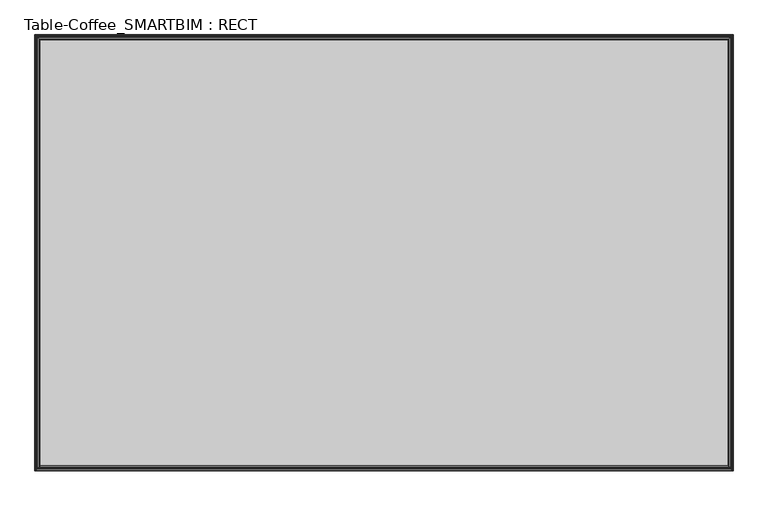
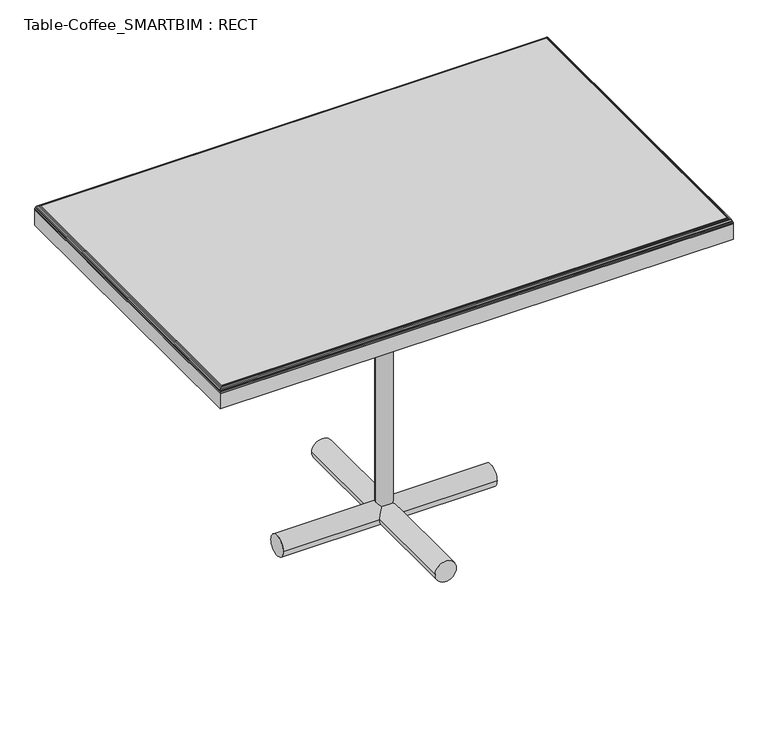
"""IFC4 building model written with IfcOpenShell, lengths in millimetres: furniture geometry, Table-Coffee_SMARTBIM : RECT."""

import ifcopenshell
import ifcopenshell.guid

model = None  # the IFC model being written
_history = None  # IfcOwnerHistory: only IFC2X3 demands one
_inside = {}  # id of a spatial element -> (the spatial element, [elements in it])
_under = {}  # id of a project, library or spatial element -> (it, [spatial elements below it])
_declared = {}  # id of a project -> (the project, [libraries it declares])
_typed = {}  # id of a type object -> (the type object, [elements of that type])
_made_of = {}  # id of a material, layer set ... -> (it, [elements and type objects made of it])


def new_model(schema):
    """Start an empty IFC model of exactly this schema.

    Asked for "IFC4X3", IfcOpenShell would pick the latest addendum, in which some entities
    have other attributes; the version numbers below select the first issue.
    IFC2X3 requires an IfcOwnerHistory on every rooted entity: one is made here for all.
    """
    global model, _history
    if schema == "IFC4X3":
        model = ifcopenshell.file(schema_version=(4, 3, 0, 0))
    else:
        model = ifcopenshell.file(schema=schema)
    _inside.clear()
    _under.clear()
    _declared.clear()
    _typed.clear()
    _made_of.clear()
    _history = None
    if model.schema == "IFC2X3":
        org = make("IfcOrganization", Name="unknown")
        user = make(
            "IfcPersonAndOrganization",
            ThePerson=make("IfcPerson", FamilyName="unknown"),
            TheOrganization=org,
        )
        app = make(
            "IfcApplication",
            ApplicationDeveloper=org,
            Version="unknown",
            ApplicationFullName="unknown",
            ApplicationIdentifier="unknown",
        )
        _history = make(
            "IfcOwnerHistory",
            OwningUser=user,
            OwningApplication=app,
            ChangeAction="ADDED",
            CreationDate=0,
        )
    return model


def make(cls, **values):
    """One entity of the class cls with the attributes given. An attribute that is None is left unset."""
    return model.create_entity(
        cls, **{name: value for name, value in values.items() if value is not None}
    )


def rooted(cls, **values):
    """An entity with a GlobalId (a new one), such as an element, a storey or a relation."""
    return make(cls, GlobalId=ifcopenshell.guid.new(), OwnerHistory=_history, **values)


def si_unit(unit_type, name, prefix=None):
    """IfcSIUnit, for example si_unit("LENGTHUNIT", "METRE", prefix="MILLI")."""
    return make("IfcSIUnit", UnitType=unit_type, Prefix=prefix, Name=name)


def assignment(units):
    """IfcUnitAssignment: the units of a project."""
    return None if units is None else make("IfcUnitAssignment", Units=units)


def point(xyz):
    """IfcCartesianPoint."""
    return None if xyz is None else make("IfcCartesianPoint", Coordinates=xyz)


def direction(xyz):
    """IfcDirection."""
    return None if xyz is None else make("IfcDirection", DirectionRatios=xyz)


def frame(location, z_axis=None, x_axis=None):
    """IfcAxis2Placement3D, a coordinate frame: its origin and axes. An axis left out is left unset."""
    return make(
        "IfcAxis2Placement3D",
        Location=point(location),
        Axis=direction(z_axis),
        RefDirection=direction(x_axis),
    )


def frame_2d(location, x_axis=None):
    """IfcAxis2Placement2D, a coordinate frame in the plane: its origin and x axis."""
    return make(
        "IfcAxis2Placement2D", Location=point(location), RefDirection=direction(x_axis)
    )


def origin():
    """The frame at (0, 0, 0) with its axes left unset."""
    return frame((0.0, 0.0, 0.0))


def origin_2d():
    """The frame at (0, 0) in the plane with its x axis left unset."""
    return frame_2d((0.0, 0.0))


def place(relative_to, where):
    """IfcLocalPlacement: puts the frame where relative to a parent placement (None: the world)."""
    return make(
        "IfcLocalPlacement", PlacementRelTo=relative_to, RelativePlacement=where
    )


def context(
    kind, dimensions, precision=None, world=None, true_north=None, identifier=None
):
    """IfcGeometricRepresentationContext, for example the 3D "Model" context."""
    return make(
        "IfcGeometricRepresentationContext",
        ContextIdentifier=identifier,
        ContextType=kind,
        CoordinateSpaceDimension=dimensions,
        Precision=precision,
        WorldCoordinateSystem=world,
        TrueNorth=true_north,
    )


def project(units=None, contexts=None):
    """IfcProject with its units and contexts."""
    return rooted(
        "IfcProject",
        Name="project",
        RepresentationContexts=contexts,
        UnitsInContext=assignment(units),
    )


def spatial(cls, under=None, at=None, **own):
    """A site, building, storey or space (cls), placed at a placement, below another one or the project."""
    s = rooted(cls, ObjectPlacement=at, **own)
    if under is not None:
        _under.setdefault(under.id(), (under, []))[1].append(s)
    return s


def polyline(points):
    """IfcPolyline through the points."""
    return make("IfcPolyline", Points=[point(p) for p in points])


def circle_curve(where, radius):
    """IfcCircle in the frame where."""
    return make("IfcCircle", Position=where, Radius=radius)


def ellipse_curve(where, semi_axis1, semi_axis2):
    """IfcEllipse in the frame where."""
    return make(
        "IfcEllipse", Position=where, SemiAxis1=semi_axis1, SemiAxis2=semi_axis2
    )


def trimmed(basis, trim1, trim2, sense, master):
    """IfcTrimmedCurve: the piece of a basis curve between two trims."""
    return make(
        "IfcTrimmedCurve",
        BasisCurve=basis,
        Trim1=trim1,
        Trim2=trim2,
        SenseAgreement=sense,
        MasterRepresentation=master,
    )


def segment(curve, same_sense, transition):
    """IfcCompositeCurveSegment."""
    return make(
        "IfcCompositeCurveSegment",
        Transition=transition,
        SameSense=same_sense,
        ParentCurve=curve,
    )


def composite_curve(segments, self_intersect=None):
    """IfcCompositeCurve: segments joined end to end."""
    return make("IfcCompositeCurve", Segments=segments, SelfIntersect=self_intersect)


def outline(outer, holes=None, kind="AREA"):
    """IfcArbitraryClosedProfileDef: a profile drawn as a closed curve; with holes, ...WithVoids."""
    if holes is None:
        return make("IfcArbitraryClosedProfileDef", ProfileType=kind, OuterCurve=outer)
    return make(
        "IfcArbitraryProfileDefWithVoids",
        ProfileType=kind,
        OuterCurve=outer,
        InnerCurves=holes,
    )


def extrude(swept, where, along, depth):
    """IfcExtrudedAreaSolid: the profile swept, set in the frame where, extruded along a direction by depth."""
    return make(
        "IfcExtrudedAreaSolid",
        SweptArea=swept,
        Position=where,
        ExtrudedDirection=direction(along),
        Depth=depth,
    )


def shape(context_of_items, identifier, shape_type, items):
    """IfcShapeRepresentation: the items that make up one representation, for example the "Body"."""
    return make(
        "IfcShapeRepresentation",
        ContextOfItems=context_of_items,
        RepresentationIdentifier=identifier,
        RepresentationType=shape_type,
        Items=items,
    )


def source(mapping_origin, context_of_items, identifier, shape_type, items):
    """IfcRepresentationMap: a shape defined once, which mapped items show again and again."""
    return make(
        "IfcRepresentationMap",
        MappingOrigin=mapping_origin,
        MappedRepresentation=shape(context_of_items, identifier, shape_type, items),
    )


def transform(
    local_origin,
    x_axis=None,
    y_axis=None,
    z_axis=None,
    scale=None,
    scale2=None,
    scale3=None,
    uniform=True,
):
    """IfcCartesianTransformationOperator3D, or its non-uniform kind. x_axis, y_axis, z_axis: its Axis1, 2, 3."""
    if uniform:
        return make(
            "IfcCartesianTransformationOperator3D",
            Axis1=direction(x_axis),
            Axis2=direction(y_axis),
            LocalOrigin=point(local_origin),
            Scale=scale,
            Axis3=direction(z_axis),
        )
    return make(
        "IfcCartesianTransformationOperator3DnonUniform",
        Axis1=direction(x_axis),
        Axis2=direction(y_axis),
        LocalOrigin=point(local_origin),
        Scale=scale,
        Axis3=direction(z_axis),
        Scale2=scale2,
        Scale3=scale3,
    )


def mapped(mapping_source, mapping_target):
    """IfcMappedItem: shows the shape of a source again, moved by a transform."""
    return make(
        "IfcMappedItem", MappingSource=mapping_source, MappingTarget=mapping_target
    )


def made_of(thing, what):
    """Note that an element or type object is made of a material, layer set ...; save() writes the relation."""
    if what is not None:
        _made_of.setdefault(what.id(), (what, []))[1].append(thing)
    return thing


def element(
    cls,
    number,
    at=None,
    inside=None,
    cuts=None,
    type_object=None,
    material=None,
    context=None,
    identifier="Body",
    shape_type=None,
    held_by="IfcProductDefinitionShape",
    body=None,
    shapes=None,
    **own,
):
    """One element of the class cls, such as IfcWall. Its Tag is "e" and its number.

    at: its placement. inside: the storey or other place that contains it. cuts: it is an
    opening in that element (IfcRelVoidsElement). A single representation is given by context,
    identifier, shape_type and body (its items); several are given by shapes. held_by: the class
    of the entity that holds the representations. save() writes the other relations.
    """
    e = rooted(cls, Tag="e%d" % number, ObjectPlacement=at, **own)
    if body is not None:
        shapes = [shape(context, identifier, shape_type, body)]
    if shapes is not None:
        e.Representation = make(held_by, Representations=shapes)
    if inside is not None:
        _inside.setdefault(inside.id(), (inside, []))[1].append(e)
    if cuts is not None:
        rooted(
            "IfcRelVoidsElement", RelatingBuildingElement=cuts, RelatedOpeningElement=e
        )
    if type_object is not None:
        _typed.setdefault(type_object.id(), (type_object, []))[1].append(e)
    return made_of(e, material)


def aggregate(whole, parts):
    """IfcRelAggregates: a whole, such as a stair, and the parts it consists of."""
    return rooted("IfcRelAggregates", RelatingObject=whole, RelatedObjects=parts)


def save(model, path):
    """Write the relations noted so far, then the file.

    IfcRelAggregates (storeys below a building ...), IfcRelContainedInSpatialStructure (elements
    in a storey), IfcRelDefinesByType, IfcRelAssociatesMaterial and IfcRelDeclares: one each for
    every whole, place, type object, material and project.
    """
    for whole, parts in _under.values():
        aggregate(whole, parts)
    for where, things in _inside.values():
        rooted(
            "IfcRelContainedInSpatialStructure",
            RelatedElements=things,
            RelatingStructure=where,
        )
    for kind, things in _typed.values():
        rooted("IfcRelDefinesByType", RelatedObjects=things, RelatingType=kind)
    for what, things in _made_of.values():
        rooted("IfcRelAssociatesMaterial", RelatedObjects=things, RelatingMaterial=what)
    for by, libraries in _declared.values():
        rooted("IfcRelDeclares", RelatingContext=by, RelatedDefinitions=libraries)
    model.write(path)


def plane_surface(at):
    """IfcPlane: the flat surface through the origin of the frame at, square to its z axis."""
    return make("IfcPlane", Position=at)


def cylinder_surface(at, radius):
    """IfcCylindricalSurface: all points at the distance radius from the z axis of the frame at."""
    return make("IfcCylindricalSurface", Position=at, Radius=radius)


def advanced_brep(points, edges, surfaces, faces):
    """IfcAdvancedBrep: a solid bounded by faces that lie on surfaces and meet in shared edges.

    An edge is (start, end): straight between two places in points (the first is 0);
    or (start, end, curve); or (start, end, curve, False) where it runs against its curve.
    A face is (place in surfaces, loops), or (place, loops, False) where it looks against
    its surface's normal. A loop lists edges by number (the first is 1), with a minus sign
    where the edge is run from its end to its start. The first loop is the outer one.
    """
    corners = [point(p) for p in points]
    vertices = [make("IfcVertexPoint", VertexGeometry=c) for c in corners]
    made = []
    for start, end, *more in edges:
        made.append(
            make(
                "IfcEdgeCurve",
                EdgeStart=vertices[start],
                EdgeEnd=vertices[end],
                EdgeGeometry=more[0] if more else make("IfcPolyline", Points=[corners[start], corners[end]]),
                SameSense=more[1] if len(more) > 1 else True,
            )
        )
    hull = []
    for where, loops, *sense in faces:
        bounds = []
        for j, loop in enumerate(loops):
            ring = [make("IfcOrientedEdge", EdgeElement=made[abs(k) - 1], Orientation=k > 0) for k in loop]
            bounds.append(
                make(
                    "IfcFaceOuterBound" if j == 0 else "IfcFaceBound",
                    Bound=make("IfcEdgeLoop", EdgeList=ring),
                    Orientation=True,
                )
            )
        hull.append(make("IfcAdvancedFace", Bounds=bounds, FaceSurface=surfaces[where], SameSense=sense[0] if sense else True))
    return make("IfcAdvancedBrep", Outer=make("IfcClosedShell", CfsFaces=hull))


def table_coffee_smartbim_rect_01a6e93b(model_context):
    return source(origin(), model_context, "Body", "SolidModel", [
        extrude(outline(composite_curve([segment(trimmed(circle_curve(frame_2d((0.0, 25.4)), 25.4), [point((25.4, 25.4))], [point((-25.4, 25.4))], False, "CARTESIAN"), True, "CONTINUOUS"), segment(trimmed(circle_curve(frame_2d((0.0, 25.4)), 25.4), [point((-25.4, 25.4))], [point((25.4, 25.4))], False, "CARTESIAN"), True, "CONTINUOUS")], self_intersect=False)), frame((-254.0, 0.0, 0.0), z_axis=(1.0, 0.0, 0.0), x_axis=(0.0, 1.0, 0.0)), (0.0, 0.0, 1.0), 508.0),
        extrude(outline(composite_curve([segment(trimmed(circle_curve(frame_2d((25.4, 0.0)), 25.4), [point((25.4, -25.4))], [point((25.4, 25.4))], False, "CARTESIAN"), True, "CONTINUOUS"), segment(trimmed(circle_curve(frame_2d((25.4, 0.0)), 25.4), [point((25.4, 25.4))], [point((25.4, -25.4))], False, "CARTESIAN"), True, "CONTINUOUS")], self_intersect=False)), frame((0.0, -254.0, 0.0), z_axis=(0.0, 1.0, 0.0), x_axis=(0.0, 0.0, 1.0)), (0.0, 0.0, 1.0), 508.0),
        extrude(outline(polyline([(609.6, 381.0), (609.6, -381.0), (-609.6, -381.0), (-609.6, 381.0), (609.6, 381.0)])), frame((0.0, 0.0, 723.9), z_axis=(0.0, 0.0, 1.0), x_axis=(1.0, 0.0, 0.0)), (0.0, 0.0, 1.0), 38.1),
        advanced_brep(
        [(-600.1998654, -371.5998654, 774.7), (600.1998654, -371.5998654, 774.7), (600.1998654, 371.5998654, 774.7), (-600.1998654, 371.5998654, 774.7), (609.6, 381.0, 762.0), (609.6, -381.0, 762.0), (-609.6, -381.0, 762.0), (-609.6, 381.0, 762.0), (-609.6, 381.0, 765.2998654), (609.6, 381.0, 765.2998654), (-609.6, -381.0, 765.2998654), (609.6, -381.0, 765.2998654), (-609.2372483, -380.6372483, 767.8860287), (-609.2372483, 380.6372483, 767.8860287), (-602.3616212, 373.7616212, 774.4480533), (-602.3616212, -373.7616212, 774.4480533), (-604.3639185, 375.7639185, 773.7273912), (-604.3639185, -375.7639185, 773.7273912), (-606.4885738, 377.8885738, 772.2866155), (-606.4885738, -377.8885738, 772.2866155), (-608.5102962, 379.9102962, 769.692959), (-608.5102962, -379.9102962, 769.692959), (609.2372483, -380.6372483, 767.8860287), (602.3616212, -373.7616212, 774.4480533), (604.3639185, -375.7639185, 773.7273912), (606.4885738, -377.8885738, 772.2866155), (608.5102962, -379.9102962, 769.692959), (609.2372483, 380.6372483, 767.8860287), (602.3616212, 373.7616212, 774.4480533), (604.3639185, 375.7639185, 773.7273912), (606.4885738, 377.8885738, 772.2866155), (608.5102962, 379.9102962, 769.692959)],
        [
            (0, 1),
            (1, 2),
            (2, 3),
            (3, 0),
            (4, 5),
            (5, 6),
            (6, 7),
            (7, 4),
            (7, 8),
            (8, 9),
            (9, 4),
            (6, 10),
            (10, 8),
            (5, 11),
            (11, 10),
            (9, 11),
            (10, 12, ellipse_curve(frame((-600.1998654, -371.5998654, 765.2998654), z_axis=(-0.7071067811865475, 0.7071067811865475, 0.0), x_axis=(-0.7071067811865474, -0.7071067811865476, 0.0)), 13.2937978, 9.4001346)),
            (12, 13),
            (13, 8, ellipse_curve(frame((-600.1998654, 371.5998654, 765.2998654), z_axis=(-0.7071067811865475, -0.7071067811865475, 0.0), x_axis=(0.7071067811865474, -0.7071067811865476, 0.0)), 13.2937978, 9.4001346)),
            (14, 15),
            (15, 0, ellipse_curve(frame((-600.1998654, -371.5998654, 765.2998654), z_axis=(-0.7071067811865475, 0.7071067811865475, 0.0), x_axis=(-0.7071067811865474, -0.7071067811865476, 0.0)), 13.2937978, 9.4001346)),
            (3, 14, ellipse_curve(frame((-600.1998654, 371.5998654, 765.2998654), z_axis=(-0.7071067811865475, -0.7071067811865475, 0.0), x_axis=(0.7071067811865474, -0.7071067811865476, 0.0)), 13.2937978, 9.4001346)),
            (14, 16, ellipse_curve(frame((-600.1998654, 371.5998654, 765.2998654), z_axis=(-0.7071067811865475, -0.7071067811865475, 0.0), x_axis=(0.7071067811865474, -0.7071067811865476, 0.0)), 13.2937978, 9.4001346)),
            (16, 17),
            (17, 15, ellipse_curve(frame((-600.1998654, -371.5998654, 765.2998654), z_axis=(-0.7071067811865475, 0.7071067811865475, 0.0), x_axis=(-0.7071067811865474, -0.7071067811865476, 0.0)), 13.2937978, 9.4001346)),
            (16, 18, ellipse_curve(frame((-600.1998654, 371.5998654, 765.2998654), z_axis=(-0.7071067811865475, -0.7071067811865475, 0.0), x_axis=(0.7071067811865474, -0.7071067811865476, 0.0)), 13.2937978, 9.4001346)),
            (18, 19),
            (19, 17, ellipse_curve(frame((-600.1998654, -371.5998654, 765.2998654), z_axis=(-0.7071067811865475, 0.7071067811865475, 0.0), x_axis=(-0.7071067811865474, -0.7071067811865476, 0.0)), 13.2937978, 9.4001346)),
            (18, 20, ellipse_curve(frame((-600.1998654, 371.5998654, 765.2998654), z_axis=(-0.7071067811865475, -0.7071067811865475, 0.0), x_axis=(0.7071067811865474, -0.7071067811865476, 0.0)), 13.2937978, 9.4001346)),
            (20, 21),
            (21, 19, ellipse_curve(frame((-600.1998654, -371.5998654, 765.2998654), z_axis=(-0.7071067811865475, 0.7071067811865475, 0.0), x_axis=(-0.7071067811865474, -0.7071067811865476, 0.0)), 13.2937978, 9.4001346)),
            (12, 21, ellipse_curve(frame((-600.1998654, -371.5998654, 765.2998654), z_axis=(-0.7071067811865475, 0.7071067811865475, 0.0), x_axis=(-0.7071067811865474, -0.7071067811865476, 0.0)), 13.2937978, 9.4001346)),
            (20, 13, ellipse_curve(frame((-600.1998654, 371.5998654, 765.2998654), z_axis=(-0.7071067811865475, -0.7071067811865475, 0.0), x_axis=(0.7071067811865474, -0.7071067811865476, 0.0)), 13.2937978, 9.4001346)),
            (11, 22, ellipse_curve(frame((600.1998654, -371.5998654, 765.2998654), z_axis=(-0.7071067811865475, -0.7071067811865475, 0.0), x_axis=(0.7071067811865476, -0.7071067811865474, 0.0)), 13.2937978, 9.4001346)),
            (22, 12),
            (15, 23),
            (23, 1, ellipse_curve(frame((600.1998654, -371.5998654, 765.2998654), z_axis=(-0.7071067811865475, -0.7071067811865475, 0.0), x_axis=(0.7071067811865476, -0.7071067811865474, 0.0)), 13.2937978, 9.4001346)),
            (17, 24),
            (24, 23, ellipse_curve(frame((600.1998654, -371.5998654, 765.2998654), z_axis=(-0.7071067811865475, -0.7071067811865475, 0.0), x_axis=(0.7071067811865476, -0.7071067811865474, 0.0)), 13.2937978, 9.4001346)),
            (19, 25),
            (25, 24, ellipse_curve(frame((600.1998654, -371.5998654, 765.2998654), z_axis=(-0.7071067811865475, -0.7071067811865475, 0.0), x_axis=(0.7071067811865476, -0.7071067811865474, 0.0)), 13.2937978, 9.4001346)),
            (21, 26),
            (26, 25, ellipse_curve(frame((600.1998654, -371.5998654, 765.2998654), z_axis=(-0.7071067811865475, -0.7071067811865475, 0.0), x_axis=(0.7071067811865476, -0.7071067811865474, 0.0)), 13.2937978, 9.4001346)),
            (22, 26, ellipse_curve(frame((600.1998654, -371.5998654, 765.2998654), z_axis=(-0.7071067811865475, -0.7071067811865475, 0.0), x_axis=(0.7071067811865476, -0.7071067811865474, 0.0)), 13.2937978, 9.4001346)),
            (9, 27, ellipse_curve(frame((600.1998654, 371.5998654, 765.2998654), z_axis=(0.7071067811865475, -0.7071067811865475, 0.0), x_axis=(0.7071067811865474, 0.7071067811865476, 0.0)), 13.2937978, 9.4001346)),
            (27, 22),
            (23, 28),
            (28, 2, ellipse_curve(frame((600.1998654, 371.5998654, 765.2998654), z_axis=(0.7071067811865475, -0.7071067811865475, 0.0), x_axis=(0.7071067811865474, 0.7071067811865476, 0.0)), 13.2937978, 9.4001346)),
            (24, 29),
            (29, 28, ellipse_curve(frame((600.1998654, 371.5998654, 765.2998654), z_axis=(0.7071067811865475, -0.7071067811865475, 0.0), x_axis=(0.7071067811865474, 0.7071067811865476, 0.0)), 13.2937978, 9.4001346)),
            (25, 30),
            (30, 29, ellipse_curve(frame((600.1998654, 371.5998654, 765.2998654), z_axis=(0.7071067811865475, -0.7071067811865475, 0.0), x_axis=(0.7071067811865474, 0.7071067811865476, 0.0)), 13.2937978, 9.4001346)),
            (26, 31),
            (31, 30, ellipse_curve(frame((600.1998654, 371.5998654, 765.2998654), z_axis=(0.7071067811865475, -0.7071067811865475, 0.0), x_axis=(0.7071067811865474, 0.7071067811865476, 0.0)), 13.2937978, 9.4001346)),
            (27, 31, ellipse_curve(frame((600.1998654, 371.5998654, 765.2998654), z_axis=(0.7071067811865475, -0.7071067811865475, 0.0), x_axis=(0.7071067811865474, 0.7071067811865476, 0.0)), 13.2937978, 9.4001346)),
            (13, 27),
            (28, 14),
            (29, 16),
            (30, 18),
            (31, 20),
        ],
        [
            plane_surface(frame((-609.6, 381.0, 774.7), z_axis=(0.0, 0.0, 1.0), x_axis=(-1.0, 0.0, 0.0))),
            plane_surface(frame((-609.6, 381.0, 762.0), z_axis=(0.0, 0.0, -1.0), x_axis=(1.0, 0.0, 0.0))),
            plane_surface(frame((609.6, 381.0, 774.7), z_axis=(0.0, 1.0, 0.0), x_axis=(0.0, 0.0, -1.0))),
            plane_surface(frame((-609.6, 381.0, 774.7), z_axis=(-1.0, 0.0, 0.0), x_axis=(0.0, 0.0, -1.0))),
            plane_surface(frame((-609.6, -381.0, 774.7), z_axis=(0.0, -1.0, 0.0), x_axis=(0.0, 0.0, -1.0))),
            plane_surface(frame((609.6, -381.0, 774.7), z_axis=(1.0, 0.0, 0.0), x_axis=(0.0, 0.0, -1.0))),
            cylinder_surface(frame((-600.1998654, 381.0, 765.2998654), z_axis=(0.0, -1.0, 0.0), x_axis=(1.0, 0.0, 0.0)), 9.4001346),
            cylinder_surface(frame((-609.6, -371.5998654, 765.2998654), z_axis=(1.0, 0.0, 0.0), x_axis=(0.0, 1.0, 0.0)), 9.4001346),
            cylinder_surface(frame((600.1998654, -381.0, 765.2998654), z_axis=(0.0, 1.0, 0.0), x_axis=(-1.0, 0.0, 0.0)), 9.4001346),
            cylinder_surface(frame((609.6, 371.5998654, 765.2998654), z_axis=(-1.0, 0.0, 0.0), x_axis=(0.0, -1.0, 0.0)), 9.4001346),
        ],
        [
            (0, [[1, 2, 3, 4]]),
            (1, [[5, 6, 7, 8]]),
            (2, [[-8, 9, 10, 11]]),
            (3, [[-7, 12, 13, -9]]),
            (4, [[-6, 14, 15, -12]]),
            (5, [[-5, -11, 16, -14]]),
            (6, [[17, 18, 19, -13]]),
            (6, [[20, 21, -4, 22]]),
            (6, [[-20, 23, 24, 25]]),
            (6, [[-24, 26, 27, 28]]),
            (6, [[-27, 29, 30, 31]]),
            (6, [[-18, 32, -30, 33]]),
            (7, [[-17, -15, 34, 35]]),
            (7, [[-21, 36, 37, -1]]),
            (7, [[-25, 38, 39, -36]]),
            (7, [[-28, 40, 41, -38]]),
            (7, [[-31, 42, 43, -40]]),
            (7, [[-32, -35, 44, -42]]),
            (8, [[-34, -16, 45, 46]]),
            (8, [[-37, 47, 48, -2]]),
            (8, [[-39, 49, 50, -47]]),
            (8, [[-41, 51, 52, -49]]),
            (8, [[-43, 53, 54, -51]]),
            (8, [[-44, -46, 55, -53]]),
            (9, [[-19, 56, -45, -10]]),
            (9, [[-22, -3, -48, 57]]),
            (9, [[-23, -57, -50, 58]]),
            (9, [[-26, -58, -52, 59]]),
            (9, [[-29, -59, -54, 60]]),
            (9, [[-33, -60, -55, -56]]),
        ],
    ),
        extrude(outline(polyline([(76.2, 76.2), (76.2, -76.2), (-76.2, -76.2), (-76.2, 76.2), (76.2, 76.2)])), frame((0.0, 0.0, 755.65), z_axis=(0.0, 0.0, 1.0), x_axis=(1.0, 0.0, 0.0)), (0.0, 0.0, 1.0), 6.35),
        extrude(outline(composite_curve([segment(trimmed(circle_curve(origin_2d(), 19.05), [point((-19.05, 0.0))], [point((19.05, 0.0))], False, "CARTESIAN"), True, "CONTINUOUS"), segment(trimmed(circle_curve(origin_2d(), 19.05), [point((19.05, 0.0))], [point((-19.05, 0.0))], False, "CARTESIAN"), True, "CONTINUOUS")], self_intersect=False)), frame((0.0, 0.0, 24.2070278), z_axis=(0.0, 0.0, 1.0), x_axis=(1.0, 0.0, 0.0)), (0.0, 0.0, 1.0), 731.4429722),
    ])


if __name__ == "__main__":
    model = new_model("IFC4")
    model_context = context("Model", 3, world=origin())
    ifc_project = project(units=[si_unit("LENGTHUNIT", "METRE", prefix="MILLI")], contexts=[model_context])
    site = spatial("IfcSite", under=ifc_project)
    building = spatial("IfcBuilding", under=site)
    placement = place(None, origin())
    table_coffee_smartbim_rect_shape = table_coffee_smartbim_rect_01a6e93b(model_context)
    element("IfcFurniture", 1, ObjectType="Table-Coffee_SMARTBIM : RECT", at=placement, inside=building, context=model_context, shape_type="MappedRepresentation", body=[
        mapped(table_coffee_smartbim_rect_shape, transform((0.0, 0.0, 0.0), x_axis=(1.0, 0.0, 0.0), y_axis=(0.0, 1.0, 0.0), z_axis=(0.0, 0.0, 1.0))),
    ])
    save(model, "model.ifc")

# Revit data of these elements
# Type "Table-Coffee_SMARTBIM : RECT"
#   Subcategory = "Table\r\n"
#   SmartBIM Object Created By = "SMARTBIM, LLC"
#   Manufacturer = "SMARTBIM"
#   Assembly Code = "E2020200"
#   95 CSI = "12500"
#   04 CSI = "12 50 00"
#   table cloth = 0' - 1 1/2"
#   Width = 4' - 0"
#   SmartBIM Object Version = 3
#   Height = 2' - 6"
#   Depth = 2' - 6"
#   Default Elevation = 4' - 0"
#   white cloth_parameter = WOOD-OAKFIRE
#   Table Unit = MET
#   Glide = none
#   Glass = none
# Element 1 (IfcFurniture, "Table-Coffee_SMARTBIM : RECT")
#   Materials on its faces: "WOOD-OAKFIRE", "MET"
# Materials
#   "WOOD-OAKFIRE": class "Wood", colour RGB 198 202 183, transparency 0, Description = "Generic wood", Cost = 0
#   "MET": class "Metal", colour RGB 189 187 185, transparency 0
